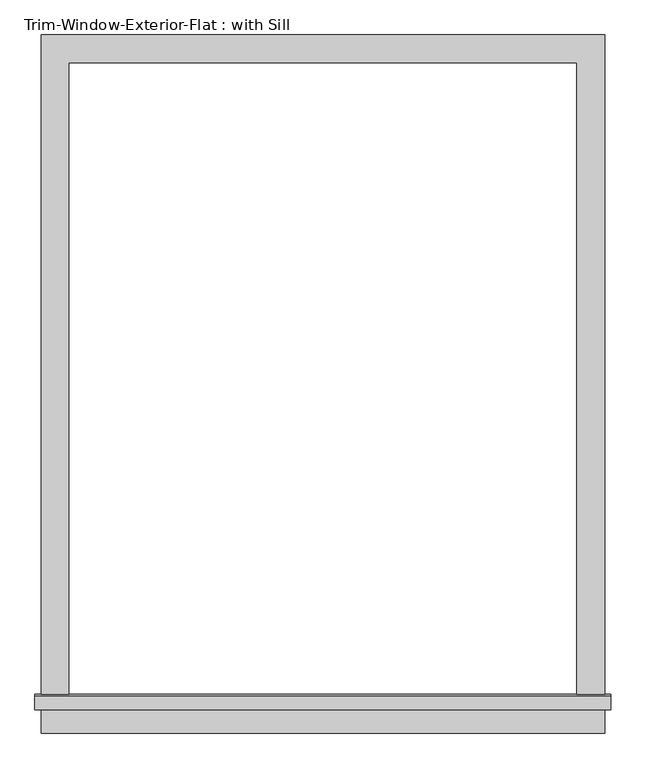
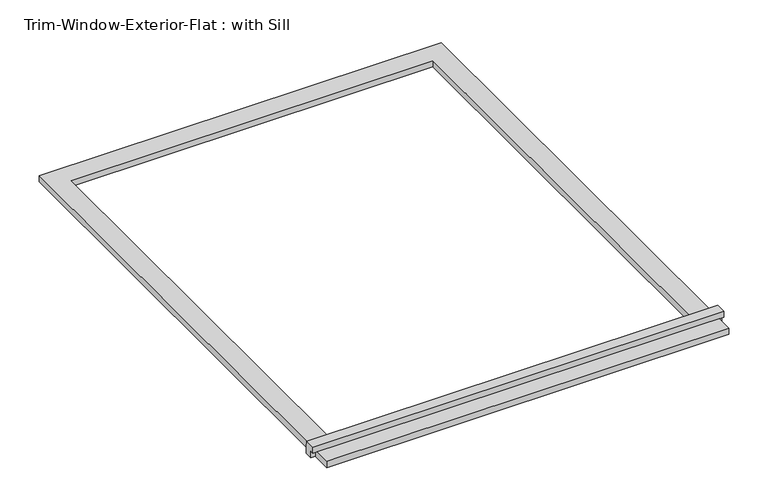
"""IFC4 building model written with IfcOpenShell, lengths in millimetres: proxy geometry, Trim-Window-Exterior-Flat : with Sill."""

from ifc_helpers import new_model, si_unit, frame, origin, origin_with_axes, place, context, project, spatial, polyline, outline, extrude, source, transform, mapped, element, save


def trim_window_exterior_flat_with_sill_39d4c871(model_context):
    return source(origin(), model_context, "Body", "SweptSolid", [
        extrude(outline(polyline([(577.85, -1317.5823709), (577.85, -1374.7323709), (-577.85, -1374.7323709), (-577.85, -1317.5823709), (577.85, -1317.5823709)])), origin_with_axes(), (0.0, 0.0, 1.0), 19.05),
        extrude(outline(polyline([(-1327.15, 38.1), (-1297.8580645, 38.1), (-1295.4, 19.05), (-1295.4, 0.0), (-1317.5823709, 0.0), (-1317.5823709, 19.05), (-1327.15, 19.05), (-1327.15, 38.1)])), frame((-590.55, 0.0, 0.0), z_axis=(1.0, 0.0, 0.0), x_axis=(0.0, 1.0, 0.0)), (0.0, 0.0, 1.0), 1181.1),
        extrude(outline(polyline([(-577.85, 57.15), (577.85, 57.15), (577.85, -1295.4), (520.7, -1295.4), (520.7, 0.0), (-520.7, 0.0), (-520.7, -1295.4), (-577.85, -1295.4), (-577.85, 57.15)])), origin_with_axes(), (0.0, 0.0, 1.0), 19.05),
    ])


if __name__ == "__main__":
    model = new_model("IFC4")
    model_context = context("Model", 3, world=origin())
    ifc_project = project(units=[si_unit("LENGTHUNIT", "METRE", prefix="MILLI")], contexts=[model_context])
    site = spatial("IfcSite", under=ifc_project)
    building = spatial("IfcBuilding", under=site)
    placement = place(None, origin())
    trim_window_exterior_flat_with_sill_shape = trim_window_exterior_flat_with_sill_39d4c871(model_context)
    element("IfcBuildingElementProxy", 1, Name="Trim-Window-Exterior-Flat : with Sill", ObjectType="Trim-Window-Exterior-Flat : with Sill", at=placement, inside=building, context=model_context, shape_type="MappedRepresentation", body=[
        mapped(trim_window_exterior_flat_with_sill_shape, transform((0.0, 0.0, 0.0), x_axis=(1.0, 0.0, 0.0), y_axis=(0.0, 1.0, 0.0), z_axis=(0.0, 0.0, 1.0))),
    ])
    save(model, "model.ifc")

# Revit data of these elements
# Type "Trim-Window-Exterior-Flat : with Sill"
#   Trim Width = 0' - 2 1/4"
#   Trim Thickness_Picture Frame = 0' - 1 1/4"
#   Trim Thickness_with Sill = 0' - 0 3/4"
#   Sill Thickness = 0' - 1 1/4"
#   Opening Width [instance default] = 2' - 0"
#   Opening Height [instance default] = 3' - 0"
#   Default Elevation = 4' - 0"
#   Sill = yes
#   Picture Frame = no
#   Trim Material [instance default] = none
# Element 1 (IfcBuildingElementProxy, "Trim-Window-Exterior-Flat : with Sill")
#   Opening Width = 3' - 5"
#   Opening Height = 4' - 3"
#   Trim Material = 1X WOOD COMPOSITE TRIM
#   Materials on its faces: "1X WOOD COMPOSITE TRIM"
# Materials
#   "1X WOOD COMPOSITE TRIM": class "Generic", colour RGB 88 61 61, transparency 0, Cost = 0
